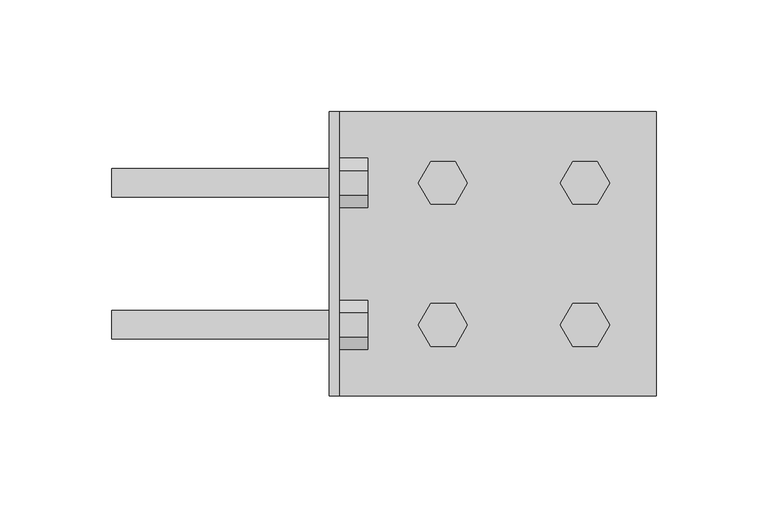
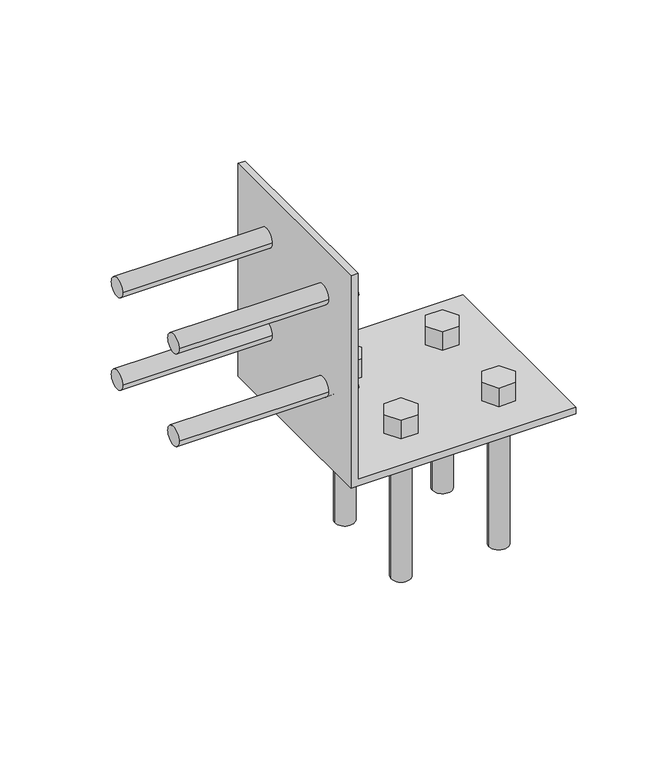
"""IFC4 building model written with IfcOpenShell, lengths in millimetres: fastener geometry."""

import ifcopenshell
import ifcopenshell.guid

model = None  # the IFC model being written
_history = None  # IfcOwnerHistory: only IFC2X3 demands one
_inside = {}  # id of a spatial element -> (the spatial element, [elements in it])
_under = {}  # id of a project, library or spatial element -> (it, [spatial elements below it])
_declared = {}  # id of a project -> (the project, [libraries it declares])
_typed = {}  # id of a type object -> (the type object, [elements of that type])
_made_of = {}  # id of a material, layer set ... -> (it, [elements and type objects made of it])


def new_model(schema):
    """Start an empty IFC model of exactly this schema.

    Asked for "IFC4X3", IfcOpenShell would pick the latest addendum, in which some entities
    have other attributes; the version numbers below select the first issue.
    IFC2X3 requires an IfcOwnerHistory on every rooted entity: one is made here for all.
    """
    global model, _history
    if schema == "IFC4X3":
        model = ifcopenshell.file(schema_version=(4, 3, 0, 0))
    else:
        model = ifcopenshell.file(schema=schema)
    _inside.clear()
    _under.clear()
    _declared.clear()
    _typed.clear()
    _made_of.clear()
    _history = None
    if model.schema == "IFC2X3":
        org = make("IfcOrganization", Name="unknown")
        user = make(
            "IfcPersonAndOrganization",
            ThePerson=make("IfcPerson", FamilyName="unknown"),
            TheOrganization=org,
        )
        app = make(
            "IfcApplication",
            ApplicationDeveloper=org,
            Version="unknown",
            ApplicationFullName="unknown",
            ApplicationIdentifier="unknown",
        )
        _history = make(
            "IfcOwnerHistory",
            OwningUser=user,
            OwningApplication=app,
            ChangeAction="ADDED",
            CreationDate=0,
        )
    return model


def make(cls, **values):
    """One entity of the class cls with the attributes given. An attribute that is None is left unset."""
    return model.create_entity(
        cls, **{name: value for name, value in values.items() if value is not None}
    )


def rooted(cls, **values):
    """An entity with a GlobalId (a new one), such as an element, a storey or a relation."""
    return make(cls, GlobalId=ifcopenshell.guid.new(), OwnerHistory=_history, **values)


def si_unit(unit_type, name, prefix=None):
    """IfcSIUnit, for example si_unit("LENGTHUNIT", "METRE", prefix="MILLI")."""
    return make("IfcSIUnit", UnitType=unit_type, Prefix=prefix, Name=name)


def assignment(units):
    """IfcUnitAssignment: the units of a project."""
    return None if units is None else make("IfcUnitAssignment", Units=units)


def point(xyz):
    """IfcCartesianPoint."""
    return None if xyz is None else make("IfcCartesianPoint", Coordinates=xyz)


def direction(xyz):
    """IfcDirection."""
    return None if xyz is None else make("IfcDirection", DirectionRatios=xyz)


def frame(location, z_axis=None, x_axis=None):
    """IfcAxis2Placement3D, a coordinate frame: its origin and axes. An axis left out is left unset."""
    return make(
        "IfcAxis2Placement3D",
        Location=point(location),
        Axis=direction(z_axis),
        RefDirection=direction(x_axis),
    )


def frame_2d(location, x_axis=None):
    """IfcAxis2Placement2D, a coordinate frame in the plane: its origin and x axis."""
    return make(
        "IfcAxis2Placement2D", Location=point(location), RefDirection=direction(x_axis)
    )


def origin():
    """The frame at (0, 0, 0) with its axes left unset."""
    return frame((0.0, 0.0, 0.0))


def place(relative_to, where):
    """IfcLocalPlacement: puts the frame where relative to a parent placement (None: the world)."""
    return make(
        "IfcLocalPlacement", PlacementRelTo=relative_to, RelativePlacement=where
    )


def context(
    kind, dimensions, precision=None, world=None, true_north=None, identifier=None
):
    """IfcGeometricRepresentationContext, for example the 3D "Model" context."""
    return make(
        "IfcGeometricRepresentationContext",
        ContextIdentifier=identifier,
        ContextType=kind,
        CoordinateSpaceDimension=dimensions,
        Precision=precision,
        WorldCoordinateSystem=world,
        TrueNorth=true_north,
    )


def project(units=None, contexts=None):
    """IfcProject with its units and contexts."""
    return rooted(
        "IfcProject",
        Name="project",
        RepresentationContexts=contexts,
        UnitsInContext=assignment(units),
    )


def spatial(cls, under=None, at=None, **own):
    """A site, building, storey or space (cls), placed at a placement, below another one or the project."""
    s = rooted(cls, ObjectPlacement=at, **own)
    if under is not None:
        _under.setdefault(under.id(), (under, []))[1].append(s)
    return s


def polyline(points):
    """IfcPolyline through the points."""
    return make("IfcPolyline", Points=[point(p) for p in points])


def circle_curve(where, radius):
    """IfcCircle in the frame where."""
    return make("IfcCircle", Position=where, Radius=radius)


def trimmed(basis, trim1, trim2, sense, master):
    """IfcTrimmedCurve: the piece of a basis curve between two trims."""
    return make(
        "IfcTrimmedCurve",
        BasisCurve=basis,
        Trim1=trim1,
        Trim2=trim2,
        SenseAgreement=sense,
        MasterRepresentation=master,
    )


def segment(curve, same_sense, transition):
    """IfcCompositeCurveSegment."""
    return make(
        "IfcCompositeCurveSegment",
        Transition=transition,
        SameSense=same_sense,
        ParentCurve=curve,
    )


def composite_curve(segments, self_intersect=None):
    """IfcCompositeCurve: segments joined end to end."""
    return make("IfcCompositeCurve", Segments=segments, SelfIntersect=self_intersect)


def outline(outer, holes=None, kind="AREA"):
    """IfcArbitraryClosedProfileDef: a profile drawn as a closed curve; with holes, ...WithVoids."""
    if holes is None:
        return make("IfcArbitraryClosedProfileDef", ProfileType=kind, OuterCurve=outer)
    return make(
        "IfcArbitraryProfileDefWithVoids",
        ProfileType=kind,
        OuterCurve=outer,
        InnerCurves=holes,
    )


def extrude(swept, where, along, depth):
    """IfcExtrudedAreaSolid: the profile swept, set in the frame where, extruded along a direction by depth."""
    return make(
        "IfcExtrudedAreaSolid",
        SweptArea=swept,
        Position=where,
        ExtrudedDirection=direction(along),
        Depth=depth,
    )


def shape(context_of_items, identifier, shape_type, items):
    """IfcShapeRepresentation: the items that make up one representation, for example the "Body"."""
    return make(
        "IfcShapeRepresentation",
        ContextOfItems=context_of_items,
        RepresentationIdentifier=identifier,
        RepresentationType=shape_type,
        Items=items,
    )


def source(mapping_origin, context_of_items, identifier, shape_type, items):
    """IfcRepresentationMap: a shape defined once, which mapped items show again and again."""
    return make(
        "IfcRepresentationMap",
        MappingOrigin=mapping_origin,
        MappedRepresentation=shape(context_of_items, identifier, shape_type, items),
    )


def transform(
    local_origin,
    x_axis=None,
    y_axis=None,
    z_axis=None,
    scale=None,
    scale2=None,
    scale3=None,
    uniform=True,
):
    """IfcCartesianTransformationOperator3D, or its non-uniform kind. x_axis, y_axis, z_axis: its Axis1, 2, 3."""
    if uniform:
        return make(
            "IfcCartesianTransformationOperator3D",
            Axis1=direction(x_axis),
            Axis2=direction(y_axis),
            LocalOrigin=point(local_origin),
            Scale=scale,
            Axis3=direction(z_axis),
        )
    return make(
        "IfcCartesianTransformationOperator3DnonUniform",
        Axis1=direction(x_axis),
        Axis2=direction(y_axis),
        LocalOrigin=point(local_origin),
        Scale=scale,
        Axis3=direction(z_axis),
        Scale2=scale2,
        Scale3=scale3,
    )


def mapped(mapping_source, mapping_target):
    """IfcMappedItem: shows the shape of a source again, moved by a transform."""
    return make(
        "IfcMappedItem", MappingSource=mapping_source, MappingTarget=mapping_target
    )


def made_of(thing, what):
    """Note that an element or type object is made of a material, layer set ...; save() writes the relation."""
    if what is not None:
        _made_of.setdefault(what.id(), (what, []))[1].append(thing)
    return thing


def element(
    cls,
    number,
    at=None,
    inside=None,
    cuts=None,
    type_object=None,
    material=None,
    context=None,
    identifier="Body",
    shape_type=None,
    held_by="IfcProductDefinitionShape",
    body=None,
    shapes=None,
    **own,
):
    """One element of the class cls, such as IfcWall. Its Tag is "e" and its number.

    at: its placement. inside: the storey or other place that contains it. cuts: it is an
    opening in that element (IfcRelVoidsElement). A single representation is given by context,
    identifier, shape_type and body (its items); several are given by shapes. held_by: the class
    of the entity that holds the representations. save() writes the other relations.
    """
    e = rooted(cls, Tag="e%d" % number, ObjectPlacement=at, **own)
    if body is not None:
        shapes = [shape(context, identifier, shape_type, body)]
    if shapes is not None:
        e.Representation = make(held_by, Representations=shapes)
    if inside is not None:
        _inside.setdefault(inside.id(), (inside, []))[1].append(e)
    if cuts is not None:
        rooted(
            "IfcRelVoidsElement", RelatingBuildingElement=cuts, RelatedOpeningElement=e
        )
    if type_object is not None:
        _typed.setdefault(type_object.id(), (type_object, []))[1].append(e)
    return made_of(e, material)


def aggregate(whole, parts):
    """IfcRelAggregates: a whole, such as a stair, and the parts it consists of."""
    return rooted("IfcRelAggregates", RelatingObject=whole, RelatedObjects=parts)


def save(model, path):
    """Write the relations noted so far, then the file.

    IfcRelAggregates (storeys below a building ...), IfcRelContainedInSpatialStructure (elements
    in a storey), IfcRelDefinesByType, IfcRelAssociatesMaterial and IfcRelDeclares: one each for
    every whole, place, type object, material and project.
    """
    for whole, parts in _under.values():
        aggregate(whole, parts)
    for where, things in _inside.values():
        rooted(
            "IfcRelContainedInSpatialStructure",
            RelatedElements=things,
            RelatingStructure=where,
        )
    for kind, things in _typed.values():
        rooted("IfcRelDefinesByType", RelatedObjects=things, RelatingType=kind)
    for what, things in _made_of.values():
        rooted("IfcRelAssociatesMaterial", RelatedObjects=things, RelatingMaterial=what)
    for by, libraries in _declared.values():
        rooted("IfcRelDeclares", RelatingContext=by, RelatedDefinitions=libraries)
    model.write(path)


def plane_surface(at):
    """IfcPlane: the flat surface through the origin of the frame at, square to its z axis."""
    return make("IfcPlane", Position=at)


def revolved_surface(curve, axis_point, axis_direction):
    """IfcSurfaceOfRevolution: the curve turned about the line through axis_point along axis_direction."""
    return make(
        "IfcSurfaceOfRevolution",
        SweptCurve=make("IfcArbitraryOpenProfileDef", ProfileType="CURVE", Curve=curve),
        AxisPosition=make("IfcAxis1Placement", Location=point(axis_point), Axis=direction(axis_direction)),
    )


def advanced_brep(points, edges, surfaces, faces):
    """IfcAdvancedBrep: a solid bounded by faces that lie on surfaces and meet in shared edges.

    An edge is (start, end): straight between two places in points (the first is 0);
    or (start, end, curve); or (start, end, curve, False) where it runs against its curve.
    A face is (place in surfaces, loops), or (place, loops, False) where it looks against
    its surface's normal. A loop lists edges by number (the first is 1), with a minus sign
    where the edge is run from its end to its start. The first loop is the outer one.
    """
    corners = [point(p) for p in points]
    vertices = [make("IfcVertexPoint", VertexGeometry=c) for c in corners]
    made = []
    for start, end, *more in edges:
        made.append(
            make(
                "IfcEdgeCurve",
                EdgeStart=vertices[start],
                EdgeEnd=vertices[end],
                EdgeGeometry=more[0] if more else make("IfcPolyline", Points=[corners[start], corners[end]]),
                SameSense=more[1] if len(more) > 1 else True,
            )
        )
    hull = []
    for where, loops, *sense in faces:
        bounds = []
        for j, loop in enumerate(loops):
            ring = [make("IfcOrientedEdge", EdgeElement=made[abs(k) - 1], Orientation=k > 0) for k in loop]
            bounds.append(
                make(
                    "IfcFaceOuterBound" if j == 0 else "IfcFaceBound",
                    Bound=make("IfcEdgeLoop", EdgeList=ring),
                    Orientation=True,
                )
            )
        hull.append(make("IfcAdvancedFace", Bounds=bounds, FaceSurface=surfaces[where], SameSense=sense[0] if sense else True))
    return make("IfcAdvancedBrep", Outer=make("IfcClosedShell", CfsFaces=hull))


def fastener_5634bf7e(model_context):
    return source(origin(), model_context, "Body", "SolidModel", [
        extrude(outline(composite_curve([segment(trimmed(circle_curve(frame_2d((-31.75, 50.8)), 6.35), [point((-38.1, 50.8))], [point((-25.4, 50.8))], False, "CARTESIAN"), True, "CONTINUOUS"), segment(trimmed(circle_curve(frame_2d((-31.75, 50.8)), 6.35), [point((-25.4, 50.8))], [point((-38.1, 50.8))], False, "CARTESIAN"), True, "CONTINUOUS")], self_intersect=False)), frame((-97.0359375, 0.0, 0.0), z_axis=(1.0, 0.0, 0.0), x_axis=(0.0, 1.0, 0.0)), (0.0, 0.0, 1.0), 101.6),
        extrude(outline(polyline([(-42.7485226, 50.8), (-37.2492613, 60.325), (-26.2507387, 60.325), (-20.7514774, 50.8), (-26.2507387, 41.275), (-37.2492613, 41.275), (-42.7485226, 50.8)])), frame((4.5640625, 0.0, 0.0), z_axis=(1.0, 0.0, 0.0), x_axis=(0.0, 1.0, 0.0)), (0.0, 0.0, 1.0), 12.7),
        extrude(outline(composite_curve([segment(trimmed(circle_curve(frame_2d((31.75, 50.8)), 6.35), [point((25.4, 50.8))], [point((38.1, 50.8))], False, "CARTESIAN"), True, "CONTINUOUS"), segment(trimmed(circle_curve(frame_2d((31.75, 50.8)), 6.35), [point((38.1, 50.8))], [point((25.4, 50.8))], False, "CARTESIAN"), True, "CONTINUOUS")], self_intersect=False)), frame((-97.0359375, 0.0, 0.0), z_axis=(1.0, 0.0, 0.0), x_axis=(0.0, 1.0, 0.0)), (0.0, 0.0, 1.0), 101.6),
        extrude(outline(polyline([(20.7514774, 50.8), (26.2507387, 60.325), (37.2492613, 60.325), (42.7485226, 50.8), (37.2492613, 41.275), (26.2507387, 41.275), (20.7514774, 50.8)])), frame((4.5640625, 0.0, 0.0), z_axis=(1.0, 0.0, 0.0), x_axis=(0.0, 1.0, 0.0)), (0.0, 0.0, 1.0), 12.7),
        extrude(outline(composite_curve([segment(trimmed(circle_curve(frame_2d((31.75, 114.3)), 6.35), [point((25.4, 114.3))], [point((38.1, 114.3))], False, "CARTESIAN"), True, "CONTINUOUS"), segment(trimmed(circle_curve(frame_2d((31.75, 114.3)), 6.35), [point((38.1, 114.3))], [point((25.4, 114.3))], False, "CARTESIAN"), True, "CONTINUOUS")], self_intersect=False)), frame((-97.0359375, 0.0, 0.0), z_axis=(1.0, 0.0, 0.0), x_axis=(0.0, 1.0, 0.0)), (0.0, 0.0, 1.0), 101.6),
        extrude(outline(polyline([(20.7514774, 114.3), (26.2507387, 123.825), (37.2492613, 123.825), (42.7485226, 114.3), (37.2492613, 104.775), (26.2507387, 104.775), (20.7514774, 114.3)])), frame((4.5640625, 0.0, 0.0), z_axis=(1.0, 0.0, 0.0), x_axis=(0.0, 1.0, 0.0)), (0.0, 0.0, 1.0), 12.7),
        extrude(outline(composite_curve([segment(trimmed(circle_curve(frame_2d((-31.75, 114.3)), 6.35), [point((-38.1, 114.3))], [point((-25.4, 114.3))], False, "CARTESIAN"), True, "CONTINUOUS"), segment(trimmed(circle_curve(frame_2d((-31.75, 114.3)), 6.35), [point((-25.4, 114.3))], [point((-38.1, 114.3))], False, "CARTESIAN"), True, "CONTINUOUS")], self_intersect=False)), frame((-97.0359375, 0.0, 0.0), z_axis=(1.0, 0.0, 0.0), x_axis=(0.0, 1.0, 0.0)), (0.0, 0.0, 1.0), 101.6),
        extrude(outline(polyline([(-42.7485226, 114.3), (-37.2492613, 123.825), (-26.2507387, 123.825), (-20.7514774, 114.3), (-26.2507387, 104.775), (-37.2492613, 104.775), (-42.7485226, 114.3)])), frame((4.5640625, 0.0, 0.0), z_axis=(1.0, 0.0, 0.0), x_axis=(0.0, 1.0, 0.0)), (0.0, 0.0, 1.0), 12.7),
        extrude(outline(composite_curve([segment(trimmed(circle_curve(frame_2d((50.8, 31.75)), 6.35), [point((44.45, 31.75))], [point((57.15, 31.75))], False, "CARTESIAN"), True, "CONTINUOUS"), segment(trimmed(circle_curve(frame_2d((50.8, 31.75)), 6.35), [point((57.15, 31.75))], [point((44.45, 31.75))], False, "CARTESIAN"), True, "CONTINUOUS")], self_intersect=False)), frame((0.0, 0.0, -97.0359375), z_axis=(0.0, 0.0, 1.0), x_axis=(1.0, 0.0, 0.0)), (0.0, 0.0, 1.0), 101.6),
        extrude(outline(polyline([(39.8014774, 31.75), (45.3007387, 41.275), (56.2992613, 41.275), (61.7985226, 31.75), (56.2992613, 22.225), (45.3007387, 22.225), (39.8014774, 31.75)])), frame((0.0, 0.0, 4.5640625), z_axis=(0.0, 0.0, 1.0), x_axis=(1.0, 0.0, 0.0)), (0.0, 0.0, 1.0), 12.7),
        extrude(outline(composite_curve([segment(trimmed(circle_curve(frame_2d((114.3, 31.75)), 6.35), [point((107.95, 31.75))], [point((120.65, 31.75))], False, "CARTESIAN"), True, "CONTINUOUS"), segment(trimmed(circle_curve(frame_2d((114.3, 31.75)), 6.35), [point((120.65, 31.75))], [point((107.95, 31.75))], False, "CARTESIAN"), True, "CONTINUOUS")], self_intersect=False)), frame((0.0, 0.0, -97.0359375), z_axis=(0.0, 0.0, 1.0), x_axis=(1.0, 0.0, 0.0)), (0.0, 0.0, 1.0), 101.6),
        extrude(outline(polyline([(103.3014774, 31.75), (108.8007387, 41.275), (119.7992613, 41.275), (125.2985226, 31.75), (119.7992613, 22.225), (108.8007387, 22.225), (103.3014774, 31.75)])), frame((0.0, 0.0, 4.5640625), z_axis=(0.0, 0.0, 1.0), x_axis=(1.0, 0.0, 0.0)), (0.0, 0.0, 1.0), 12.7),
        extrude(outline(composite_curve([segment(trimmed(circle_curve(frame_2d((114.3, -31.75)), 6.35), [point((107.95, -31.75))], [point((120.65, -31.75))], False, "CARTESIAN"), True, "CONTINUOUS"), segment(trimmed(circle_curve(frame_2d((114.3, -31.75)), 6.35), [point((120.65, -31.75))], [point((107.95, -31.75))], False, "CARTESIAN"), True, "CONTINUOUS")], self_intersect=False)), frame((0.0, 0.0, -97.0359375), z_axis=(0.0, 0.0, 1.0), x_axis=(1.0, 0.0, 0.0)), (0.0, 0.0, 1.0), 101.6),
        extrude(outline(polyline([(103.3014774, -31.75), (108.8007387, -22.225), (119.7992613, -22.225), (125.2985226, -31.75), (119.7992613, -41.275), (108.8007387, -41.275), (103.3014774, -31.75)])), frame((0.0, 0.0, 4.5640625), z_axis=(0.0, 0.0, 1.0), x_axis=(1.0, 0.0, 0.0)), (0.0, 0.0, 1.0), 12.7),
        extrude(outline(composite_curve([segment(trimmed(circle_curve(frame_2d((50.8, -31.75)), 6.35), [point((44.45, -31.75))], [point((57.15, -31.75))], False, "CARTESIAN"), True, "CONTINUOUS"), segment(trimmed(circle_curve(frame_2d((50.8, -31.75)), 6.35), [point((57.15, -31.75))], [point((44.45, -31.75))], False, "CARTESIAN"), True, "CONTINUOUS")], self_intersect=False)), frame((0.0, 0.0, -97.0359375), z_axis=(0.0, 0.0, 1.0), x_axis=(1.0, 0.0, 0.0)), (0.0, 0.0, 1.0), 101.6),
        extrude(outline(polyline([(39.8014774, -31.75), (45.3007387, -22.225), (56.2992613, -22.225), (61.7985226, -31.75), (56.2992613, -41.275), (45.3007387, -41.275), (39.8014774, -31.75)])), frame((0.0, 0.0, 4.5640625), z_axis=(0.0, 0.0, 1.0), x_axis=(1.0, 0.0, 0.0)), (0.0, 0.0, 1.0), 12.7),
        advanced_brep(
        [(4.5640625, 63.5, 146.05), (4.5640625, -63.5, 146.05), (4.5640625, -63.5, 4.5640625), (4.5640625, 63.5, 4.5640625), (4.5640625, -25.4, 50.8), (4.5640625, -38.1, 50.8), (4.5640625, 38.1, 50.8), (4.5640625, 25.4, 50.8), (4.5640625, 38.1, 114.3), (4.5640625, 25.4, 114.3), (4.5640625, -25.4, 114.3), (4.5640625, -38.1, 114.3), (0.0, -63.5, 146.05), (0.0, 63.5, 146.05), (0.0, 63.5, 0.0), (0.0, -63.5, 0.0), (0.0, -38.1, 50.8), (0.0, -25.4, 50.8), (0.0, 25.4, 50.8), (0.0, 38.1, 50.8), (0.0, 25.4, 114.3), (0.0, 38.1, 114.3), (0.0, -38.1, 114.3), (0.0, -25.4, 114.3), (146.05, -63.5, 0.0), (146.05, -63.5, 4.5640625), (146.05, 63.5, 4.5640625), (146.05, 63.5, 0.0), (57.15, -31.75, 4.5640625), (44.45, -31.75, 4.5640625), (120.65, -31.75, 4.5640625), (107.95, -31.75, 4.5640625), (57.15, 31.75, 4.5640625), (44.45, 31.75, 4.5640625), (120.65, 31.75, 4.5640625), (107.95, 31.75, 4.5640625), (44.45, -31.75, 0.0), (57.15, -31.75, 0.0), (107.95, -31.75, 0.0), (120.65, -31.75, 0.0), (44.45, 31.75, 0.0), (57.15, 31.75, 0.0), (107.95, 31.75, 0.0), (120.65, 31.75, 0.0)],
        [
            (0, 1),
            (1, 2),
            (2, 3),
            (3, 0),
            (4, 5, circle_curve(frame((4.5640625, -31.75, 50.8), z_axis=(-1.0, 0.0, 0.0), x_axis=(0.0, 1.0, 0.0)), 6.35)),
            (5, 4, circle_curve(frame((4.5640625, -31.75, 50.8), z_axis=(-1.0, 0.0, 0.0), x_axis=(0.0, 1.0, 0.0)), 6.35)),
            (6, 7, circle_curve(frame((4.5640625, 31.75, 50.8), z_axis=(-1.0, 0.0, 0.0), x_axis=(0.0, 1.0, 0.0)), 6.35)),
            (7, 6, circle_curve(frame((4.5640625, 31.75, 50.8), z_axis=(-1.0, 0.0, 0.0), x_axis=(0.0, 1.0, 0.0)), 6.35)),
            (8, 9, circle_curve(frame((4.5640625, 31.75, 114.3), z_axis=(-1.0, 0.0, 0.0), x_axis=(0.0, 1.0, 0.0)), 6.35)),
            (9, 8, circle_curve(frame((4.5640625, 31.75, 114.3), z_axis=(-1.0, 0.0, 0.0), x_axis=(0.0, 1.0, 0.0)), 6.35)),
            (10, 11, circle_curve(frame((4.5640625, -31.75, 114.3), z_axis=(-1.0, 0.0, 0.0), x_axis=(0.0, 1.0, 0.0)), 6.35)),
            (11, 10, circle_curve(frame((4.5640625, -31.75, 114.3), z_axis=(-1.0, 0.0, 0.0), x_axis=(0.0, 1.0, 0.0)), 6.35)),
            (12, 13),
            (13, 14),
            (14, 15),
            (15, 12),
            (16, 17, circle_curve(frame((0.0, -31.75, 50.8), z_axis=(1.0, 0.0, 0.0), x_axis=(0.0, 1.0, 0.0)), 6.35)),
            (17, 16, circle_curve(frame((0.0, -31.75, 50.8), z_axis=(1.0, 0.0, 0.0), x_axis=(0.0, 1.0, 0.0)), 6.35)),
            (18, 19, circle_curve(frame((0.0, 31.75, 50.8), z_axis=(1.0, 0.0, 0.0), x_axis=(0.0, 1.0, 0.0)), 6.35)),
            (19, 18, circle_curve(frame((0.0, 31.75, 50.8), z_axis=(1.0, 0.0, 0.0), x_axis=(0.0, 1.0, 0.0)), 6.35)),
            (20, 21, circle_curve(frame((0.0, 31.75, 114.3), z_axis=(1.0, 0.0, 0.0), x_axis=(0.0, 1.0, 0.0)), 6.35)),
            (21, 20, circle_curve(frame((0.0, 31.75, 114.3), z_axis=(1.0, 0.0, 0.0), x_axis=(0.0, 1.0, 0.0)), 6.35)),
            (22, 23, circle_curve(frame((0.0, -31.75, 114.3), z_axis=(1.0, 0.0, 0.0), x_axis=(0.0, 1.0, 0.0)), 6.35)),
            (23, 22, circle_curve(frame((0.0, -31.75, 114.3), z_axis=(1.0, 0.0, 0.0), x_axis=(0.0, 1.0, 0.0)), 6.35)),
            (0, 13),
            (12, 1),
            (15, 24),
            (24, 25),
            (25, 2),
            (3, 26),
            (26, 27),
            (27, 14),
            (25, 26),
            (28, 29, circle_curve(frame((50.8, -31.75, 4.5640625), z_axis=(0.0, 0.0, -1.0), x_axis=(1.0, 0.0, 0.0)), 6.35)),
            (29, 28, circle_curve(frame((50.8, -31.75, 4.5640625), z_axis=(0.0, 0.0, -1.0), x_axis=(1.0, 0.0, 0.0)), 6.35)),
            (30, 31, circle_curve(frame((114.3, -31.75, 4.5640625), z_axis=(0.0, 0.0, -1.0), x_axis=(1.0, 0.0, 0.0)), 6.35)),
            (31, 30, circle_curve(frame((114.3, -31.75, 4.5640625), z_axis=(0.0, 0.0, -1.0), x_axis=(1.0, 0.0, 0.0)), 6.35)),
            (32, 33, circle_curve(frame((50.8, 31.75, 4.5640625), z_axis=(0.0, 0.0, -1.0), x_axis=(1.0, 0.0, 0.0)), 6.35)),
            (33, 32, circle_curve(frame((50.8, 31.75, 4.5640625), z_axis=(0.0, 0.0, -1.0), x_axis=(1.0, 0.0, 0.0)), 6.35)),
            (34, 35, circle_curve(frame((114.3, 31.75, 4.5640625), z_axis=(0.0, 0.0, -1.0), x_axis=(1.0, 0.0, 0.0)), 6.35)),
            (35, 34, circle_curve(frame((114.3, 31.75, 4.5640625), z_axis=(0.0, 0.0, -1.0), x_axis=(1.0, 0.0, 0.0)), 6.35)),
            (27, 24),
            (36, 37, circle_curve(frame((50.8, -31.75, 0.0), z_axis=(0.0, 0.0, 1.0), x_axis=(1.0, 0.0, 0.0)), 6.35)),
            (37, 36, circle_curve(frame((50.8, -31.75, 0.0), z_axis=(0.0, 0.0, 1.0), x_axis=(1.0, 0.0, 0.0)), 6.35)),
            (38, 39, circle_curve(frame((114.3, -31.75, 0.0), z_axis=(0.0, 0.0, 1.0), x_axis=(1.0, 0.0, 0.0)), 6.35)),
            (39, 38, circle_curve(frame((114.3, -31.75, 0.0), z_axis=(0.0, 0.0, 1.0), x_axis=(1.0, 0.0, 0.0)), 6.35)),
            (40, 41, circle_curve(frame((50.8, 31.75, 0.0), z_axis=(0.0, 0.0, 1.0), x_axis=(1.0, 0.0, 0.0)), 6.35)),
            (41, 40, circle_curve(frame((50.8, 31.75, 0.0), z_axis=(0.0, 0.0, 1.0), x_axis=(1.0, 0.0, 0.0)), 6.35)),
            (42, 43, circle_curve(frame((114.3, 31.75, 0.0), z_axis=(0.0, 0.0, 1.0), x_axis=(1.0, 0.0, 0.0)), 6.35)),
            (43, 42, circle_curve(frame((114.3, 31.75, 0.0), z_axis=(0.0, 0.0, 1.0), x_axis=(1.0, 0.0, 0.0)), 6.35)),
            (28, 37),
            (36, 29),
            (38, 31),
            (30, 39),
            (40, 33),
            (32, 41),
            (42, 35),
            (34, 43),
            (4, 17),
            (16, 5),
            (18, 7),
            (6, 19),
            (20, 9),
            (8, 21),
            (22, 11),
            (10, 23),
        ],
        [
            plane_surface(frame((4.5640625, -63.5, 146.05), z_axis=(1.0, 0.0, 0.0), x_axis=(0.0, -1.0, 0.0))),
            plane_surface(frame((0.0, -63.5, 146.05), z_axis=(-1.0, 0.0, 0.0), x_axis=(0.0, 1.0, 0.0))),
            plane_surface(frame((4.5640625, 63.5, 146.05), z_axis=(0.0, 0.0, 1.0), x_axis=(-1.0, 0.0, 0.0))),
            plane_surface(frame((4.5640625, -63.5, 146.05), z_axis=(0.0, -1.0, 0.0), x_axis=(-1.0, 0.0, 0.0))),
            plane_surface(frame((4.5640625, 63.5, 4.5640625), z_axis=(0.0, 1.0, 0.0), x_axis=(-1.0, 0.0, 0.0))),
            plane_surface(frame((0.0, 63.5, 4.5640625), z_axis=(0.0, 0.0, 1.0), x_axis=(-1.0, 0.0, 0.0))),
            plane_surface(frame((0.0, 63.5, 0.0), z_axis=(0.0, 0.0, -1.0), x_axis=(1.0, 0.0, 0.0))),
            plane_surface(frame((146.05, -63.5, 4.5640625), z_axis=(1.0, 0.0, 0.0), x_axis=(0.0, 0.0, -1.0))),
            revolved_surface(polyline([(57.15, -31.75, 4.5640625), (57.15, -31.75, 0.0)]), (50.8, -31.75, 0.0), (0.0, 0.0, 1.0)),
            revolved_surface(polyline([(120.64999999999999, -31.75, 4.5640625), (120.64999999999999, -31.75, 0.0)]), (114.3, -31.75, 0.0), (0.0, 0.0, 1.0)),
            revolved_surface(polyline([(57.15, 31.75, 4.5640625), (57.15, 31.75, 0.0)]), (50.8, 31.75, 0.0), (0.0, 0.0, 1.0)),
            revolved_surface(polyline([(120.64999999999999, 31.75, 4.5640625), (120.64999999999999, 31.75, 0.0)]), (114.3, 31.75, 0.0), (0.0, 0.0, 1.0)),
            revolved_surface(polyline([(4.5640625, -25.4, 50.8), (0.0, -25.4, 50.8)]), (0.0, -31.75, 50.8), (1.0, 0.0, 0.0)),
            revolved_surface(polyline([(4.5640625, 38.1, 50.8), (0.0, 38.1, 50.8)]), (0.0, 31.75, 50.8), (1.0, 0.0, 0.0)),
            revolved_surface(polyline([(4.5640625, 38.1, 114.3), (0.0, 38.1, 114.3)]), (0.0, 31.75, 114.3), (1.0, 0.0, 0.0)),
            revolved_surface(polyline([(4.5640625, -25.4, 114.3), (0.0, -25.4, 114.3)]), (0.0, -31.75, 114.3), (1.0, 0.0, 0.0)),
        ],
        [
            (0, [[1, 2, 3, 4], [5, 6], [7, 8], [9, 10], [11, 12]]),
            (1, [[13, 14, 15, 16], [17, 18], [19, 20], [21, 22], [23, 24]]),
            (2, [[-1, 25, -13, 26]]),
            (3, [[-2, -26, -16, 27, 28, 29]]),
            (4, [[-4, 30, 31, 32, -14, -25]]),
            (5, [[33, -30, -3, -29], [34, 35], [36, 37], [38, 39], [40, 41]]),
            (6, [[42, -27, -15, -32], [43, 44], [45, 46], [47, 48], [49, 50]]),
            (7, [[-33, -28, -42, -31]]),
            (8, [[51, -43, 52, -34]]),
            (8, [[-51, -35, -52, -44]]),
            (9, [[53, -36, 54, -45]]),
            (9, [[-53, -46, -54, -37]]),
            (10, [[55, -38, 56, -47]]),
            (10, [[-55, -48, -56, -39]]),
            (11, [[57, -40, 58, -49]]),
            (11, [[-57, -50, -58, -41]]),
            (12, [[59, -17, 60, -5]]),
            (12, [[-59, -6, -60, -18]]),
            (13, [[61, -7, 62, -19]]),
            (13, [[-61, -20, -62, -8]]),
            (14, [[63, -9, 64, -21]]),
            (14, [[-63, -22, -64, -10]]),
            (15, [[65, -11, 66, -23]]),
            (15, [[-65, -24, -66, -12]]),
        ],
    ),
    ])


if __name__ == "__main__":
    model = new_model("IFC4")
    model_context = context("Model", 3, world=origin())
    ifc_project = project(units=[si_unit("LENGTHUNIT", "METRE", prefix="MILLI")], contexts=[model_context])
    site = spatial("IfcSite", under=ifc_project)
    building = spatial("IfcBuilding", under=site)
    placement = place(None, origin())
    fastener_shape = fastener_5634bf7e(model_context)
    element("IfcFastener", 1, ObjectType="060523 - W_P_C - Fastenings - Simpson - HLGPC Heavy Angles and Gussets : SIMPSON -HL55 - 5 X 5.75 - .5\" BOLT - HDG", at=placement, inside=building, context=model_context, shape_type="MappedRepresentation", body=[
        mapped(fastener_shape, transform((0.0, 0.0, 0.0), x_axis=(1.0, 0.0, 0.0), y_axis=(0.0, 1.0, 0.0), z_axis=(0.0, 0.0, 1.0))),
    ])
    save(model, "model.ifc")

# Revit data of these elements
# Type "060523 - W_P_C - Fastenings - Simpson - HLGPC Heavy Angles and Gussets : SIMPSON -HL55 - 5 X 5.75 - .5\" BOLT - HDG"
#   URL = "https://www.strongtie.com/classiccollection_architecturalproductsgroup/hlpc-hlgpc_productgroup_wcc/p/hlpc.hlgpc"
#   L = 0' - 5"
#   Hole Radius = 0' - 0 1/4"
#   D4 = 0' - 2 1/2"
#   D2 = 0' - 2 1/2"
#   D1 = 0' - 1 1/4"
#   D3 = 0' - 2"
#   Ga. = 0' - 0 23/128"
#   W1 & W2 = 0' - 5 3/4"
#   Default Elevation = 4' - 0"
#   Bolt Visibility - 3B = no
#   Bolt Visibility - 3A = no
#   Bolt Visibility - 2B = yes
#   Bolt Visibility - 2A = yes
#   Bolt Visibility - 1B = yes
#   Bolt Visibility - 1A = yes
#   Bolt Visibility = yes
#   Bolt Size = element 1473756
# Element 1 (IfcFastener, "060523 - W_P_C - Fastenings - Simpson - HLGPC Heavy Angles and Gussets : SIMPSON -HL55 - 5 X 5.75 - .5\" BOLT - HDG")
#   Materials on its faces: "THRU-BOLT OR LAG BOLT", "SIMPSON -HL55 - 5 X 5.75 - .5\" BOLT (3 GA - RAW STEEL - NO FINISH)"
# Materials
#   "THRU-BOLT OR LAG BOLT": class "Generic", colour RGB 120 120 120, transparency 0, Cost = 0
#   "SIMPSON -HL55 - 5 X 5.75 - .5\" BOLT (3 GA - RAW STEEL - NO FINISH)": class "Generic", colour RGB 120 120 120, transparency 0, Cost = 0
